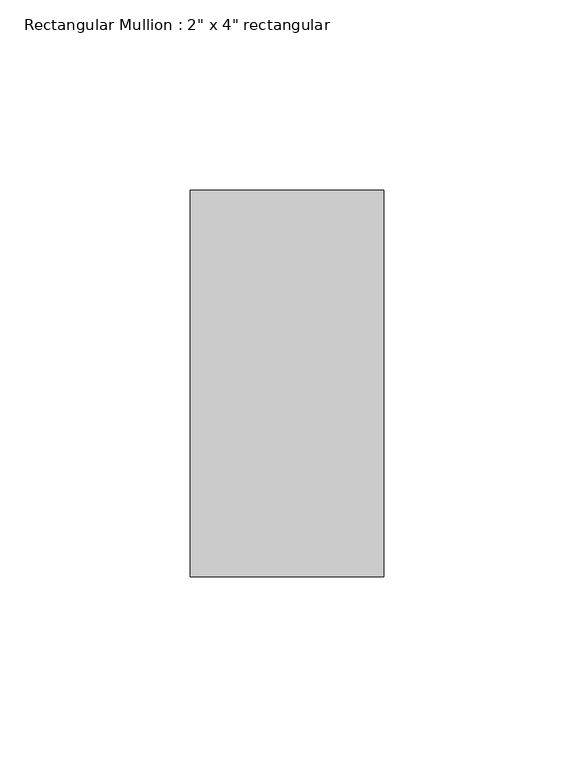
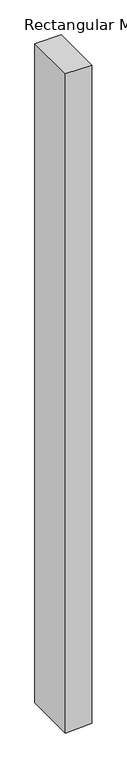
"""IFC4 building model written with IfcOpenShell, lengths in millimetres: member geometry."""

from ifc_helpers import new_model, si_unit, frame, origin, place, context, project, spatial, polyline, outline, extrude, source, transform, mapped, element, save


def member_bcb395ca(model_context):
    return source(origin(), model_context, "Body", "SweptSolid", [
        extrude(outline(polyline([(0.0, 25.4), (0.0, -25.4), (-1341.6777726, -25.4), (-1340.7075573, -2.1148317), (-1339.5611059, 25.4), (0.0, 25.4)])), frame((0.0, -50.8, 0.0), z_axis=(0.0, 1.0, 0.0), x_axis=(0.0, 0.0, 1.0)), (0.0, 0.0, 1.0), 101.6),
    ])


if __name__ == "__main__":
    model = new_model("IFC4")
    model_context = context("Model", 3, world=origin())
    ifc_project = project(units=[si_unit("LENGTHUNIT", "METRE", prefix="MILLI")], contexts=[model_context])
    site = spatial("IfcSite", under=ifc_project)
    building = spatial("IfcBuilding", under=site)
    placement = place(None, origin())
    member_shape = member_bcb395ca(model_context)
    element("IfcMember", 1, ObjectType="Rectangular Mullion : 2\" x 4\" rectangular", at=placement, inside=building, context=model_context, shape_type="MappedRepresentation", body=[
        mapped(member_shape, transform((0.0, 0.0, 0.0), x_axis=(1.0, 0.0, 0.0), y_axis=(0.0, 1.0, 0.0), z_axis=(0.0, 0.0, 1.0))),
    ])
    save(model, "model.ifc")

# Revit data of these elements
# Type "Rectangular Mullion : 2\" x 4\" rectangular"
#   built-in parameter 1007304 = 0.333333 (stored number, unit not read)
#   built-in parameter 1007301 = 0.0833333 (stored number, unit not read)
#   built-in parameter 1007300 = 0.0833333 (stored number, unit not read)
# Element 1 (IfcMember, "Rectangular Mullion : 2\" x 4\" rectangular")
#   Materials on its faces: "PAINTED STEEL C CHANNEL"
# Materials
#   "PAINTED STEEL C CHANNEL": class "Generic", colour RGB 88 62 61, transparency 0, Cost = 0
